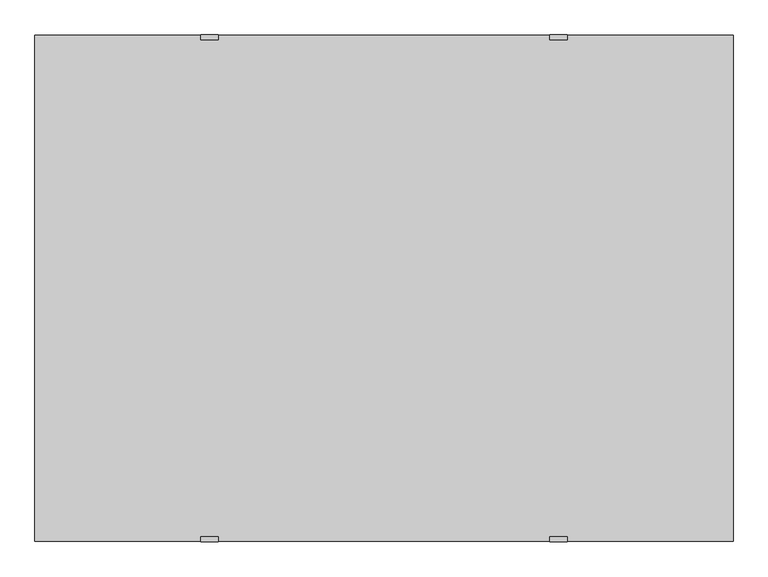
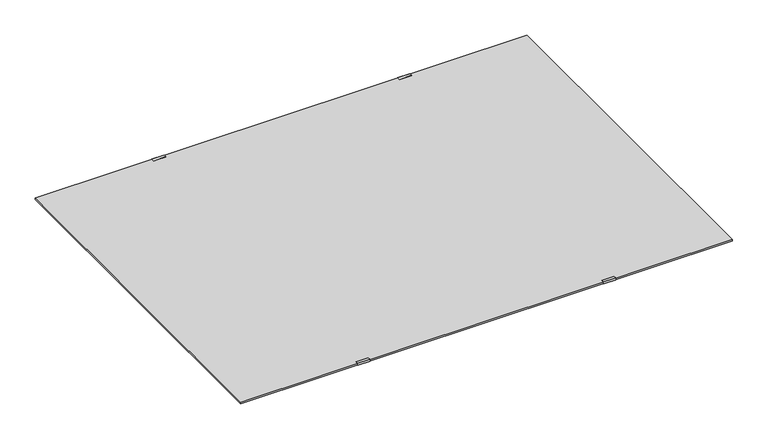
"""IFC4 building model written with IfcOpenShell, lengths in millimetres: proxy geometry."""

from ifc_helpers import new_model, si_unit, frame, origin, origin_with_axes, place, context, project, spatial, polyline, outline, extrude, source, transform, mapped, element, save


def specialty_equipment_0b5badc8(model_context):
    return source(origin(), model_context, "Body", "SweptSolid", [
        extrude(outline(polyline([(-736.6, 6.35), (-736.6, 0.0), (-737.39375, 0.0), (-737.39375, 7.14375), (-723.9, 7.14375), (-723.9, 6.35), (-736.6, 6.35)])), frame((482.6, 0.0, 0.0), z_axis=(1.0, 0.0, 0.0), x_axis=(0.0, 1.0, 0.0)), (0.0, 0.0, 1.0), 50.8),
        extrude(outline(polyline([(-736.6, 6.35), (-736.6, 0.0), (-737.39375, 0.0), (-737.39375, 7.14375), (-723.9, 7.14375), (-723.9, 6.35), (-736.6, 6.35)])), frame((-533.4, 0.0, 0.0), z_axis=(1.0, 0.0, 0.0), x_axis=(0.0, 1.0, 0.0)), (0.0, 0.0, 1.0), 50.8),
        extrude(outline(polyline([(736.6, 6.35), (723.9, 6.35), (723.9, 7.14375), (737.39375, 7.14375), (737.39375, 0.0), (736.6, 0.0), (736.6, 6.35)])), frame((482.6, 0.0, 0.0), z_axis=(1.0, 0.0, 0.0), x_axis=(0.0, 1.0, 0.0)), (0.0, 0.0, 1.0), 50.8),
        extrude(outline(polyline([(736.6, 6.35), (723.9, 6.35), (723.9, 7.14375), (737.39375, 7.14375), (737.39375, 0.0), (736.6, 0.0), (736.6, 6.35)])), frame((-533.4, 0.0, 0.0), z_axis=(1.0, 0.0, 0.0), x_axis=(0.0, 1.0, 0.0)), (0.0, 0.0, 1.0), 50.8),
        extrude(outline(polyline([(1016.0, 736.6), (1016.0, -736.6), (-1016.0, -736.6), (-1016.0, 736.6), (1016.0, 736.6)])), origin_with_axes(), (0.0, 0.0, 1.0), 6.35),
    ])


if __name__ == "__main__":
    model = new_model("IFC4")
    model_context = context("Model", 3, world=origin())
    ifc_project = project(units=[si_unit("LENGTHUNIT", "METRE", prefix="MILLI")], contexts=[model_context])
    site = spatial("IfcSite", under=ifc_project)
    building = spatial("IfcBuilding", under=site)
    placement = place(None, origin())
    specialty_equipment_shape = specialty_equipment_0b5badc8(model_context)
    element("IfcBuildingElementProxy", 1, Name="Bradley-Washroom_Accessories-Mirrors-747_Standard : 60\" x 36\" + BradEX", ObjectType="Bradley-Washroom_Accessories-Mirrors-747_Standard : 60\" x 36\" + BradEX", at=placement, inside=building, context=model_context, shape_type="MappedRepresentation", body=[
        mapped(specialty_equipment_shape, transform((0.0, 0.0, 0.0), x_axis=(1.0, 0.0, 0.0), y_axis=(0.0, 1.0, 0.0), z_axis=(0.0, 0.0, 1.0))),
    ])
    save(model, "model.ifc")

# Revit data of these elements
# Type "Bradley-Washroom_Accessories-Mirrors-747_Standard : 60\" x 36\" + BradEX"
#   Keynote = "M08831300.01"
#   Warranty Information = "Complete unit, excepting mirrors warranted for one year.\r\n Stainless steel mirror frames for fifteen years.\r\n Plate glass mirrors for fifteen years.\r\n This warranty does not cover installation or any other labor charges and does not apply to any units,\r\n which have been damaged by accident, abuse, improper installation, improper maintenance, or altered in any way."
#   Version = "1.0"
#   URL = "http://www.bradleycorp.com/"
#   Type Comments = "BradEX 1/4\" Float Glass Mirror"
#   OmniClass Title = "Mirrors"
#   OmniClass Code = "23.40.95.17.17"
#   Modeling Code = ""
#   Model = "747-024360"
#   MasterFormat Title = "Commercial Toilet Accessories"
#   MasterFormat Number = "10 28 13. 13"
#   Manufacturer = "Bradley Corporation"
#   Industry Standards = "ASTM C 1036"
#   Fire Rating = "n/a"
#   Description = "Frameless Mirror, Clip Fasteners, 24 by 36 inches"
#   Copyright = "This Model Data is Property of Bradley Corporation"
#   Buy American Act = "Yes"
#   Assembly Code = "C1030900"
#   ADA Compliant = "Yes"
#   Width = 6' - 8"
#   Height = 4' - 10"
#   Fastener Placement = 1' - 8"
#   Depth = 0' - 0 1/4"
#   Default Elevation = 3' - 4"
#   Reflective Material = Glass - Bradley Corp - BradEX - Polished Float Mirror
#   Frame Material = Bradley Corp Stainless Steel - Satin
# Element 1 (IfcBuildingElementProxy, "Bradley-Washroom_Accessories-Mirrors-747_Standard : 60\" x 36\" + BradEX")
#   Materials on its faces: "Bradley Corp Stainless Steel - Satin", "Glass - Bradley Corp - BradEX - Polished Float Mirror"
# Materials
#   "Glass - Bradley Corp - BradEX - Polished Float Mirror": class "Glass", colour RGB 221 230 232, transparency 0, Manufacturer = "Bradley Corporation", URL = "www.bradleycorp.com", Description = "Stainless Steel - Satin Finish", Cost = 0
#   "Bradley Corp Stainless Steel - Satin": class "Metal", colour RGB 189 187 185, transparency 0, Manufacturer = "Bradley Corporation", URL = "www.bradleycorp.com", Description = "Stainless Steel - Satin Finish", Cost = 0
